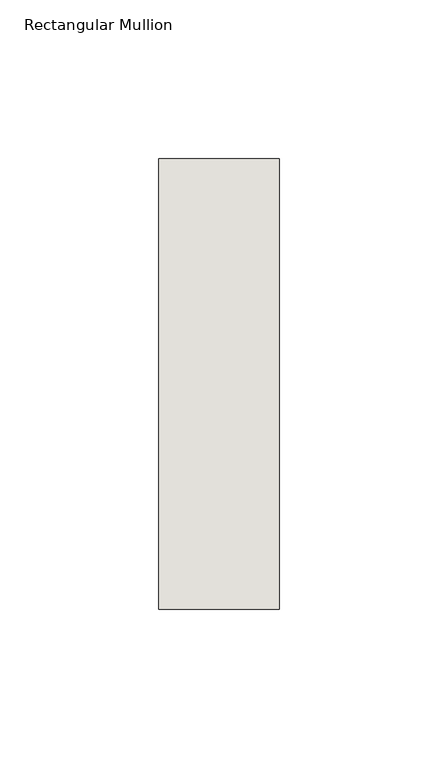
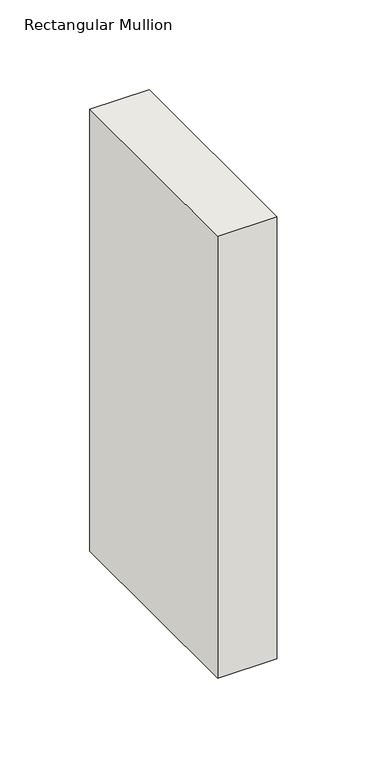
"""IFC4 building model written with IfcOpenShell, lengths in millimetres: wall geometry, Rectangular Mullion : NLRS_21_CWM_hsb-regel 38x142_gen_rsf."""

from ifc_helpers import new_model, si_unit, frame, origin, place, context, project, spatial, polyline, outline, extrude, source, transform, mapped, element, save


def rectangular_mullion_8803486b(model_context):
    return source(origin(), model_context, "Body", "SweptSolid", [
        extrude(outline(polyline([(0.0, -71.0), (-38.0, -71.0), (-38.0, 71.0), (0.0, 71.0), (0.0, -71.0)])), frame((0.0, 0.0, -300.0), z_axis=(0.0, 0.0, 1.0), x_axis=(1.0, 0.0, 0.0)), (0.0, 0.0, 1.0), 300.0),
    ])


if __name__ == "__main__":
    model = new_model("IFC4")
    model_context = context("Model", 3, world=origin())
    ifc_project = project(units=[si_unit("LENGTHUNIT", "METRE", prefix="MILLI")], contexts=[model_context])
    site = spatial("IfcSite", under=ifc_project)
    building = spatial("IfcBuilding", under=site)
    placement = place(None, origin())
    rectangular_mullion_shape = rectangular_mullion_8803486b(model_context)
    element("IfcWall", 1, ObjectType="Rectangular Mullion : NLRS_21_CWM_hsb-regel 38x142_gen_rsf", at=placement, inside=building, context=model_context, shape_type="MappedRepresentation", body=[
        mapped(rectangular_mullion_shape, transform((0.0, 0.0, 0.0), x_axis=(1.0, 0.0, 0.0), y_axis=(0.0, 1.0, 0.0), z_axis=(0.0, 0.0, 1.0))),
    ])
    save(model, "model.ifc")

# Revit data of these elements
# Type "Rectangular Mullion : NLRS_21_CWM_hsb-regel 38x142_gen_rsf"
#   Type IfcGUID = "07M7mRoiH1CR8m_RSKIwpF"
#   Assembly Code = "21.10"
#   IfcExportAs = "IfcWall"
#   built-in parameter 1007322 = 0.465879 (stored number, unit not read)
#   built-in parameter 1007321 = 0.062336 (stored number, unit not read)
#   built-in parameter 1007320 = 0.062336 (stored number, unit not read)
# Element 1 (IfcWall, "Rectangular Mullion : NLRS_21_CWM_hsb-regel 38x142_gen_rsf")
#   Materials on its faces: "NLRS_i2_hout naaldhout vuren_gen_rsf"
# Materials
#   "NLRS_i2_hout naaldhout vuren_gen_rsf": class "I - Hout", colour RGB 234 199 147, transparency 0, Keynote = "i2", Manufacturer = "Revit Standards Foundation", URL = "www.revitstandards.org", Description = "hout vuren", Cost = 0
